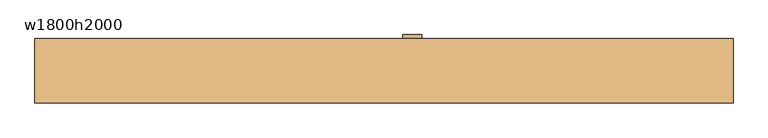
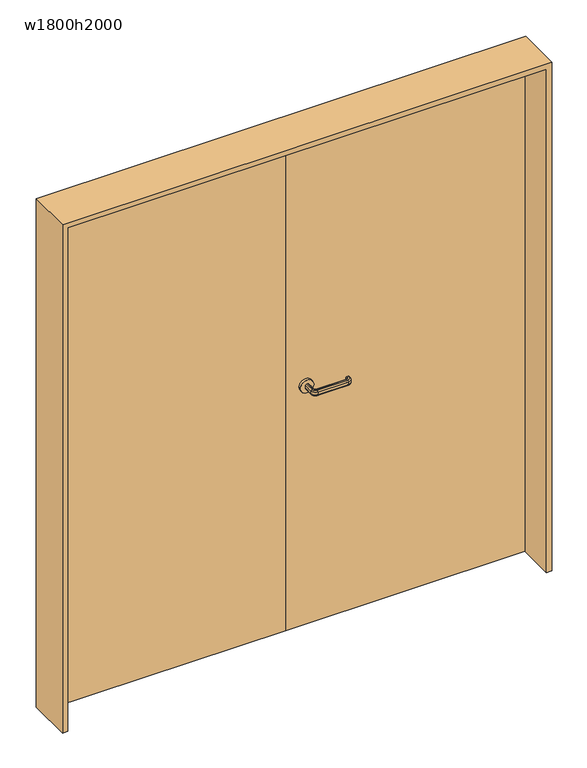
"""IFC4 building model written with IfcOpenShell, lengths in millimetres: door geometry, 二重 : w1800h2000."""

from ifc_helpers import new_model, si_unit, point, frame, frame_2d, origin, origin_with_axes, place, context, project, spatial, polyline, circle_curve, ellipse_curve, trimmed, segment, composite_curve, outline, extrude, source, transform, mapped, element, save
from ifc_brep_helpers import plane_surface, cylinder_surface, revolved_surface, advanced_brep


def w1800h2000_7614bfdb(model_context):
    return source(origin(), model_context, "Body", "SolidModel", [
        advanced_brep(
        [(77.0, 45.0, 940.0), (73.0, 45.0, 940.0), (68.0, 45.0, 945.0), (68.0, 45.0, 955.0), (73.0, 45.0, 960.0), (77.0, 45.0, 960.0), (82.0, 45.0, 955.0), (82.0, 45.0, 945.0), (77.0, 10.0, 940.0), (85.0, 2.0, 940.0), (200.0, 2.0, 940.0), (208.0, 10.0, 940.0), (208.0, 15.0, 940.0), (212.0, 15.0, 940.0), (212.0, 10.0, 940.0), (200.0, -2.0, 940.0), (85.0, -2.0, 940.0), (73.0, 10.0, 940.0), (68.0, 10.0, 945.0), (68.0, 10.0, 955.0), (73.0, 10.0, 960.0), (85.0, -2.0, 960.0), (200.0, -2.0, 960.0), (212.0, 10.0, 960.0), (212.0, 15.0, 960.0), (208.0, 15.0, 960.0), (208.0, 10.0, 960.0), (200.0, 2.0, 960.0), (85.0, 2.0, 960.0), (77.0, 10.0, 960.0), (82.0, 10.0, 955.0), (82.0, 10.0, 945.0), (85.0, -7.0, 945.0), (85.0, -7.0, 955.0), (85.0, 7.0, 955.0), (85.0, 7.0, 945.0), (200.0, -7.0, 945.0), (200.0, -7.0, 955.0), (200.0, 7.0, 955.0), (200.0, 7.0, 945.0), (217.0, 10.0, 945.0), (217.0, 10.0, 955.0), (203.0, 10.0, 955.0), (203.0, 10.0, 945.0), (203.0, 15.0, 945.0), (203.0, 15.0, 955.0), (217.0, 15.0, 955.0), (217.0, 15.0, 945.0)],
        [
            (0, 1),
            (1, 2, circle_curve(frame((73.0, 45.0, 945.0), z_axis=(0.0, 1.0, 0.0), x_axis=(1.0, 0.0, 0.0)), 5.0)),
            (2, 3),
            (3, 4, circle_curve(frame((73.0, 45.0, 955.0), z_axis=(0.0, 1.0, 0.0), x_axis=(1.0, 0.0, 0.0)), 5.0)),
            (4, 5),
            (5, 6, circle_curve(frame((77.0, 45.0, 955.0), z_axis=(0.0, 1.0, 0.0), x_axis=(1.0, 0.0, 0.0)), 5.0)),
            (6, 7),
            (7, 0, circle_curve(frame((77.0, 45.0, 945.0), z_axis=(0.0, 1.0, 0.0), x_axis=(1.0, 0.0, 0.0)), 5.0)),
            (0, 8),
            (8, 9, circle_curve(frame((85.0, 10.0, 940.0), z_axis=(0.0, 0.0, 1.0), x_axis=(-1.0, 0.0, 0.0)), 8.0)),
            (9, 10),
            (10, 11, circle_curve(frame((200.0, 10.0, 940.0), z_axis=(0.0, 0.0, 1.0), x_axis=(0.0, -1.0, 0.0)), 8.0)),
            (11, 12),
            (12, 13),
            (13, 14),
            (14, 15, circle_curve(frame((200.0, 10.0, 940.0), z_axis=(0.0, 0.0, -1.0), x_axis=(0.0, -1.0, 0.0)), 12.0)),
            (15, 16),
            (16, 17, circle_curve(frame((85.0, 10.0, 940.0), z_axis=(0.0, 0.0, -1.0), x_axis=(-1.0, 0.0, 0.0)), 12.0)),
            (17, 1),
            (17, 18, circle_curve(frame((73.0, 10.0, 945.0), z_axis=(0.0, 1.0, 0.0), x_axis=(1.0, 0.0, 0.0)), 5.0)),
            (18, 2),
            (18, 19),
            (19, 3),
            (19, 20, circle_curve(frame((73.0, 10.0, 955.0), z_axis=(0.0, 1.0, 0.0), x_axis=(1.0, 0.0, 0.0)), 5.0)),
            (20, 4),
            (20, 21, circle_curve(frame((85.0, 10.0, 960.0), z_axis=(0.0, 0.0, 1.0), x_axis=(-1.0, 0.0, 0.0)), 12.0)),
            (21, 22),
            (22, 23, circle_curve(frame((200.0, 10.0, 960.0), z_axis=(0.0, 0.0, 1.0), x_axis=(0.0, -1.0, 0.0)), 12.0)),
            (23, 24),
            (24, 25),
            (25, 26),
            (26, 27, circle_curve(frame((200.0, 10.0, 960.0), z_axis=(0.0, 0.0, -1.0), x_axis=(0.0, -1.0, 0.0)), 8.0)),
            (27, 28),
            (28, 29, circle_curve(frame((85.0, 10.0, 960.0), z_axis=(0.0, 0.0, -1.0), x_axis=(-1.0, 0.0, 0.0)), 8.0)),
            (29, 5),
            (29, 30, circle_curve(frame((77.0, 10.0, 955.0), z_axis=(0.0, 1.0, 0.0), x_axis=(1.0, 0.0, 0.0)), 5.0)),
            (30, 6),
            (30, 31),
            (31, 7),
            (31, 8, circle_curve(frame((77.0, 10.0, 945.0), z_axis=(0.0, 1.0, 0.0), x_axis=(1.0, 0.0, 0.0)), 5.0)),
            (32, 18, circle_curve(frame((85.0, 10.0, 945.0), z_axis=(0.0, 0.0, -1.0), x_axis=(-1.0, 0.0, 0.0)), 17.0)),
            (16, 32, circle_curve(frame((85.0, -2.0, 945.0), z_axis=(-1.0, 0.0, 0.0), x_axis=(0.0, 1.0, 0.0)), 5.0)),
            (33, 19, circle_curve(frame((85.0, 10.0, 955.0), z_axis=(0.0, 0.0, -1.0), x_axis=(-1.0, 0.0, 0.0)), 17.0)),
            (32, 33),
            (33, 21, circle_curve(frame((85.0, -2.0, 955.0), z_axis=(-1.0, 0.0, 0.0), x_axis=(0.0, 1.0, 0.0)), 5.0)),
            (34, 30, circle_curve(frame((85.0, 10.0, 955.0), z_axis=(0.0, 0.0, -1.0), x_axis=(-1.0, 0.0, 0.0)), 3.0)),
            (28, 34, circle_curve(frame((85.0, 2.0, 955.0), z_axis=(-1.0, 0.0, 0.0), x_axis=(0.0, 1.0, 0.0)), 5.0)),
            (35, 31, circle_curve(frame((85.0, 10.0, 945.0), z_axis=(0.0, 0.0, -1.0), x_axis=(-1.0, 0.0, 0.0)), 3.0)),
            (34, 35),
            (35, 9, circle_curve(frame((85.0, 2.0, 945.0), z_axis=(-1.0, 0.0, 0.0), x_axis=(0.0, 1.0, 0.0)), 5.0)),
            (15, 36, circle_curve(frame((200.0, -2.0, 945.0), z_axis=(-1.0, 0.0, 0.0), x_axis=(0.0, 1.0, 0.0)), 5.0)),
            (36, 32),
            (36, 37),
            (37, 33),
            (37, 22, circle_curve(frame((200.0, -2.0, 955.0), z_axis=(-1.0, 0.0, 0.0), x_axis=(0.0, 1.0, 0.0)), 5.0)),
            (27, 38, circle_curve(frame((200.0, 2.0, 955.0), z_axis=(-1.0, 0.0, 0.0), x_axis=(0.0, 1.0, 0.0)), 5.0)),
            (38, 34),
            (38, 39),
            (39, 35),
            (39, 10, circle_curve(frame((200.0, 2.0, 945.0), z_axis=(-1.0, 0.0, 0.0), x_axis=(0.0, 1.0, 0.0)), 5.0)),
            (40, 36, circle_curve(frame((200.0, 10.0, 945.0), z_axis=(0.0, 0.0, -1.0), x_axis=(0.0, -1.0, 0.0)), 17.0)),
            (14, 40, circle_curve(frame((212.0, 10.0, 945.0), z_axis=(0.0, -1.0, 0.0), x_axis=(-1.0, 0.0, 0.0)), 5.0)),
            (41, 37, circle_curve(frame((200.0, 10.0, 955.0), z_axis=(0.0, 0.0, -1.0), x_axis=(0.0, -1.0, 0.0)), 17.0)),
            (40, 41),
            (41, 23, circle_curve(frame((212.0, 10.0, 955.0), z_axis=(0.0, -1.0, 0.0), x_axis=(-1.0, 0.0, 0.0)), 5.0)),
            (42, 38, circle_curve(frame((200.0, 10.0, 955.0), z_axis=(0.0, 0.0, -1.0), x_axis=(0.0, -1.0, 0.0)), 3.0)),
            (26, 42, circle_curve(frame((208.0, 10.0, 955.0), z_axis=(0.0, -1.0, 0.0), x_axis=(-1.0, 0.0, 0.0)), 5.0)),
            (43, 39, circle_curve(frame((200.0, 10.0, 945.0), z_axis=(0.0, 0.0, -1.0), x_axis=(0.0, -1.0, 0.0)), 3.0)),
            (42, 43),
            (43, 11, circle_curve(frame((208.0, 10.0, 945.0), z_axis=(0.0, -1.0, 0.0), x_axis=(-1.0, 0.0, 0.0)), 5.0)),
            (12, 44, circle_curve(frame((208.0, 15.0, 945.0), z_axis=(0.0, 1.0, 0.0), x_axis=(-1.0, 0.0, 0.0)), 5.0)),
            (44, 45),
            (45, 25, circle_curve(frame((208.0, 15.0, 955.0), z_axis=(0.0, 1.0, 0.0), x_axis=(-1.0, 0.0, 0.0)), 5.0)),
            (24, 46, circle_curve(frame((212.0, 15.0, 955.0), z_axis=(0.0, 1.0, 0.0), x_axis=(-1.0, 0.0, 0.0)), 5.0)),
            (46, 47),
            (47, 13, circle_curve(frame((212.0, 15.0, 945.0), z_axis=(0.0, 1.0, 0.0), x_axis=(-1.0, 0.0, 0.0)), 5.0)),
            (47, 40),
            (46, 41),
            (45, 42),
            (44, 43),
        ],
        [
            plane_surface(frame((64.801961, 45.0, 950.0), z_axis=(0.0, 1.0, 0.0), x_axis=(0.0, 0.0, -1.0))),
            plane_surface(frame((77.0, 45.0, 940.0), z_axis=(0.0, 0.0, -1.0), x_axis=(0.0, -1.0, 0.0))),
            cylinder_surface(frame((73.0, 45.0, 945.0), z_axis=(0.0, 1.0, 0.0), x_axis=(1.0, 0.0, 0.0)), 5.0),
            plane_surface(frame((68.0, 45.0, 945.0), z_axis=(-1.0, 0.0, 0.0), x_axis=(0.0, -1.0, 0.0))),
            cylinder_surface(frame((73.0, 45.0, 955.0), z_axis=(0.0, 1.0, 0.0), x_axis=(1.0, 0.0, 0.0)), 5.0),
            plane_surface(frame((73.0, 45.0, 960.0), z_axis=(0.0, 0.0, 1.0), x_axis=(0.0, -1.0, 0.0))),
            cylinder_surface(frame((77.0, 45.0, 955.0), z_axis=(0.0, 1.0, 0.0), x_axis=(1.0, 0.0, 0.0)), 5.0),
            plane_surface(frame((82.0, 45.0, 955.0), z_axis=(1.0, 0.0, 0.0), x_axis=(0.0, -1.0, 0.0))),
            cylinder_surface(frame((77.0, 45.0, 945.0), z_axis=(0.0, 1.0, 0.0), x_axis=(1.0, 0.0, 0.0)), 5.0),
            revolved_surface(trimmed(ellipse_curve(frame((73.0, 10.0, 945.0), z_axis=(0.0, 1.0, 0.0), x_axis=(1.0, 0.0, 0.0)), 5.0, 5.0), [point((73.0, 10.0, 940.0))], [point((68.0, 10.0, 945.0))], True, "CARTESIAN"), (85.0, 10.0, 950.0), (0.0, 0.0, 1.0)),
            cylinder_surface(frame((85.0, 10.0, 950.0), z_axis=(0.0, 0.0, 1.0), x_axis=(-1.0, 0.0, 0.0)), 17.0),
            revolved_surface(trimmed(ellipse_curve(frame((73.0, 10.0, 955.0), z_axis=(0.0, 1.0, 0.0), x_axis=(1.0, 0.0, 0.0)), 5.0, 5.0), [point((68.0, 10.0, 955.0))], [point((73.0, 10.0, 960.0))], True, "CARTESIAN"), (85.0, 10.0, 950.0), (0.0, 0.0, 1.0)),
            revolved_surface(trimmed(ellipse_curve(frame((77.0, 10.0, 955.0), z_axis=(0.0, 1.0, 0.0), x_axis=(1.0, 0.0, 0.0)), 5.0, 5.0), [point((77.0, 10.0, 960.0))], [point((82.0, 10.0, 955.0))], True, "CARTESIAN"), (85.0, 10.0, 950.0), (0.0, 0.0, 1.0)),
            revolved_surface(polyline([(82.0, 10.0, 955.0), (82.0, 10.0, 945.0)]), (85.0, 10.0, 950.0), (0.0, 0.0, 1.0)),
            revolved_surface(trimmed(ellipse_curve(frame((77.0, 10.0, 945.0), z_axis=(0.0, 1.0, 0.0), x_axis=(1.0, 0.0, 0.0)), 5.0, 5.0), [point((82.0, 10.0, 945.0))], [point((77.0, 10.0, 940.0))], True, "CARTESIAN"), (85.0, 10.0, 950.0), (0.0, 0.0, 1.0)),
            cylinder_surface(frame((85.0, -2.0, 945.0), z_axis=(-1.0, 0.0, 0.0), x_axis=(0.0, 1.0, 0.0)), 5.0),
            plane_surface(frame((85.0, -7.0, 945.0), z_axis=(0.0, -1.0, 0.0), x_axis=(1.0, 0.0, 0.0))),
            cylinder_surface(frame((85.0, -2.0, 955.0), z_axis=(-1.0, 0.0, 0.0), x_axis=(0.0, 1.0, 0.0)), 5.0),
            cylinder_surface(frame((85.0, 2.0, 955.0), z_axis=(-1.0, 0.0, 0.0), x_axis=(0.0, 1.0, 0.0)), 5.0),
            plane_surface(frame((85.0, 7.0, 955.0), z_axis=(0.0, 1.0, 0.0), x_axis=(1.0, 0.0, 0.0))),
            cylinder_surface(frame((85.0, 2.0, 945.0), z_axis=(-1.0, 0.0, 0.0), x_axis=(0.0, 1.0, 0.0)), 5.0),
            revolved_surface(trimmed(ellipse_curve(frame((200.0, -2.0, 945.0), z_axis=(-1.0, 0.0, 0.0), x_axis=(0.0, 1.0, 0.0)), 5.0, 5.0), [point((200.0, -2.0, 940.0))], [point((200.0, -7.0, 945.0))], True, "CARTESIAN"), (200.0, 10.0, 950.0), (0.0, 0.0, 1.0)),
            cylinder_surface(frame((200.0, 10.0, 950.0), z_axis=(0.0, 0.0, 1.0), x_axis=(0.0, -1.0, 0.0)), 17.0),
            revolved_surface(trimmed(ellipse_curve(frame((200.0, -2.0, 955.0), z_axis=(-1.0, 0.0, 0.0), x_axis=(0.0, 1.0, 0.0)), 5.0, 5.0), [point((200.0, -7.0, 955.0))], [point((200.0, -2.0, 960.0))], True, "CARTESIAN"), (200.0, 10.0, 950.0), (0.0, 0.0, 1.0)),
            revolved_surface(trimmed(ellipse_curve(frame((200.0, 2.0, 955.0), z_axis=(-1.0, 0.0, 0.0), x_axis=(0.0, 1.0, 0.0)), 5.0, 5.0), [point((200.0, 2.0, 960.0))], [point((200.0, 7.0, 955.0))], True, "CARTESIAN"), (200.0, 10.0, 950.0), (0.0, 0.0, 1.0)),
            revolved_surface(polyline([(200.0, 7.0, 955.0), (200.0, 7.0, 945.0)]), (200.0, 10.0, 950.0), (0.0, 0.0, 1.0)),
            revolved_surface(trimmed(ellipse_curve(frame((200.0, 2.0, 945.0), z_axis=(-1.0, 0.0, 0.0), x_axis=(0.0, 1.0, 0.0)), 5.0, 5.0), [point((200.0, 7.0, 945.0))], [point((200.0, 2.0, 940.0))], True, "CARTESIAN"), (200.0, 10.0, 950.0), (0.0, 0.0, 1.0)),
            plane_surface(frame((199.801961, 15.0, 950.0), z_axis=(0.0, 1.0, 0.0), x_axis=(0.0, 0.0, 1.0))),
            cylinder_surface(frame((212.0, 10.0, 945.0), z_axis=(0.0, -1.0, 0.0), x_axis=(-1.0, 0.0, 0.0)), 5.0),
            plane_surface(frame((217.0, 10.0, 945.0), z_axis=(1.0, 0.0, 0.0), x_axis=(0.0, 1.0, 0.0))),
            cylinder_surface(frame((212.0, 10.0, 955.0), z_axis=(0.0, -1.0, 0.0), x_axis=(-1.0, 0.0, 0.0)), 5.0),
            cylinder_surface(frame((208.0, 10.0, 955.0), z_axis=(0.0, -1.0, 0.0), x_axis=(-1.0, 0.0, 0.0)), 5.0),
            plane_surface(frame((203.0, 10.0, 955.0), z_axis=(-1.0, 0.0, 0.0), x_axis=(0.0, 1.0, 0.0))),
            cylinder_surface(frame((208.0, 10.0, 945.0), z_axis=(0.0, -1.0, 0.0), x_axis=(-1.0, 0.0, 0.0)), 5.0),
        ],
        [
            (0, [[1, 2, 3, 4, 5, 6, 7, 8]]),
            (1, [[-1, 9, 10, 11, 12, 13, 14, 15, 16, 17, 18, 19]]),
            (2, [[-2, -19, 20, 21]]),
            (3, [[-3, -21, 22, 23]]),
            (4, [[-4, -23, 24, 25]]),
            (5, [[-5, -25, 26, 27, 28, 29, 30, 31, 32, 33, 34, 35]]),
            (6, [[-6, -35, 36, 37]]),
            (7, [[-7, -37, 38, 39]]),
            (8, [[-8, -39, 40, -9]]),
            (9, [[41, -20, -18, 42]]),
            (10, [[43, -22, -41, 44]]),
            (11, [[-26, -24, -43, 45]]),
            (12, [[46, -36, -34, 47]]),
            (13, [[48, -38, -46, 49]]),
            (14, [[-10, -40, -48, 50]]),
            (15, [[-42, -17, 51, 52]]),
            (16, [[-44, -52, 53, 54]]),
            (17, [[-45, -54, 55, -27]]),
            (18, [[-47, -33, 56, 57]]),
            (19, [[-49, -57, 58, 59]]),
            (20, [[-50, -59, 60, -11]]),
            (21, [[61, -51, -16, 62]]),
            (22, [[63, -53, -61, 64]]),
            (23, [[-28, -55, -63, 65]]),
            (24, [[66, -56, -32, 67]]),
            (25, [[68, -58, -66, 69]]),
            (26, [[-12, -60, -68, 70]]),
            (27, [[71, 72, 73, -30, 74, 75, 76, -14]]),
            (28, [[-62, -15, -76, 77]]),
            (29, [[-64, -77, -75, 78]]),
            (30, [[-65, -78, -74, -29]]),
            (31, [[-67, -31, -73, 79]]),
            (32, [[-69, -79, -72, 80]]),
            (33, [[-70, -80, -71, -13]]),
        ],
    ),
        extrude(outline(composite_curve([segment(trimmed(circle_curve(frame_2d((950.0, 75.0)), 25.0), [point((950.0, 50.0))], [point((950.0, 100.0))], False, "CARTESIAN"), True, "CONTINUOUS"), segment(trimmed(circle_curve(frame_2d((950.0, 75.0)), 25.0), [point((950.0, 100.0))], [point((950.0, 50.0))], False, "CARTESIAN"), True, "CONTINUOUS")], self_intersect=False)), frame((0.0, 85.0, 0.0), z_axis=(0.0, 1.0, 0.0), x_axis=(0.0, 0.0, 1.0)), (0.0, 0.0, 1.0), 10.0),
        extrude(outline(composite_curve([segment(trimmed(circle_curve(frame_2d((950.0, 75.0)), 25.0), [point((950.0, 50.0))], [point((950.0, 100.0))], False, "CARTESIAN"), True, "CONTINUOUS"), segment(trimmed(circle_curve(frame_2d((950.0, 75.0)), 25.0), [point((950.0, 100.0))], [point((950.0, 50.0))], False, "CARTESIAN"), True, "CONTINUOUS")], self_intersect=False)), frame((0.0, 45.0, 0.0), z_axis=(0.0, 1.0, 0.0), x_axis=(0.0, 0.0, 1.0)), (0.0, 0.0, 1.0), 10.0),
        extrude(outline(polyline([(0.0, 55.0), (-900.0, 55.0), (-900.0, 85.0), (0.0, 85.0), (0.0, 55.0)])), origin_with_axes(), (0.0, 0.0, 1.0), 2000.0),
        extrude(outline(polyline([(2020.0, -920.0), (0.0, -920.0), (0.0, -900.0), (2000.0, -900.0), (2000.0, 900.0), (0.0, 900.0), (0.0, 920.0), (2020.0, 920.0), (2020.0, -920.0)])), frame((0.0, -85.0, 0.0), z_axis=(0.0, 1.0, 0.0), x_axis=(0.0, 0.0, 1.0)), (0.0, 0.0, 1.0), 170.0),
        extrude(outline(polyline([(900.0, 55.0), (0.0, 55.0), (0.0, 85.0), (900.0, 85.0), (900.0, 55.0)])), origin_with_axes(), (0.0, 0.0, 1.0), 2000.0),
    ])


if __name__ == "__main__":
    model = new_model("IFC4")
    model_context = context("Model", 3, world=origin())
    ifc_project = project(units=[si_unit("LENGTHUNIT", "METRE", prefix="MILLI")], contexts=[model_context])
    site = spatial("IfcSite", under=ifc_project)
    building = spatial("IfcBuilding", under=site)
    placement = place(None, origin())
    w1800h2000_shape = w1800h2000_7614bfdb(model_context)
    element("IfcDoor", 1, ObjectType="二重 : w1800h2000", at=placement, inside=building, context=model_context, shape_type="MappedRepresentation", body=[
        mapped(w1800h2000_shape, transform((0.0, 0.0, 0.0), x_axis=(1.0, 0.0, 0.0), y_axis=(0.0, 1.0, 0.0), z_axis=(0.0, 0.0, 1.0))),
    ])
    save(model, "model.ifc")

# Revit data of these elements
# Type "二重 : w1800h2000"
#   Construction Type Id = "MDOOR"
#   Analytic Construction = "メタル"
#   Type Mark = "45"
#   Operation = "両開きドア単一スイング"
#   Keynote = "08110.R1"
#   Visual Light Transmittance = 0
#   Solar Heat Gain Coefficient = 0
#   Heat Transfer Coefficient (U) = 3.7021 W/(m²·K)
#   高さ(中心) = 1000 mm
#   Height = 2000 mm
#   Thickness = 30 mm
#   ドア枠見附 = 20 mm
#   Width = 1800 mm
#   取手取付け高さ = 950 mm
#   ドア枠ちり = 10 mm
#   Function = 0
#   ドア枠 [instance default] = none
#   ドア把手 [instance default] = メタル-ステンレス
#   ドア [instance default] = none
#   Wall Closure = (empty or 0)
# Element 1 (IfcDoor, "二重 : w1800h2000")
#   Materials on its faces: "メタル-ステンレス"
# Materials
#   "メタル-ステンレス": class "メタル", colour RGB 247 247 247, transparency 0, Cost = 0
